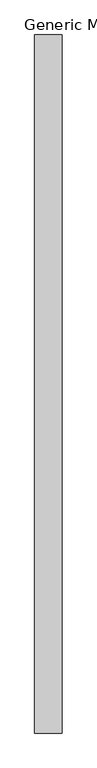
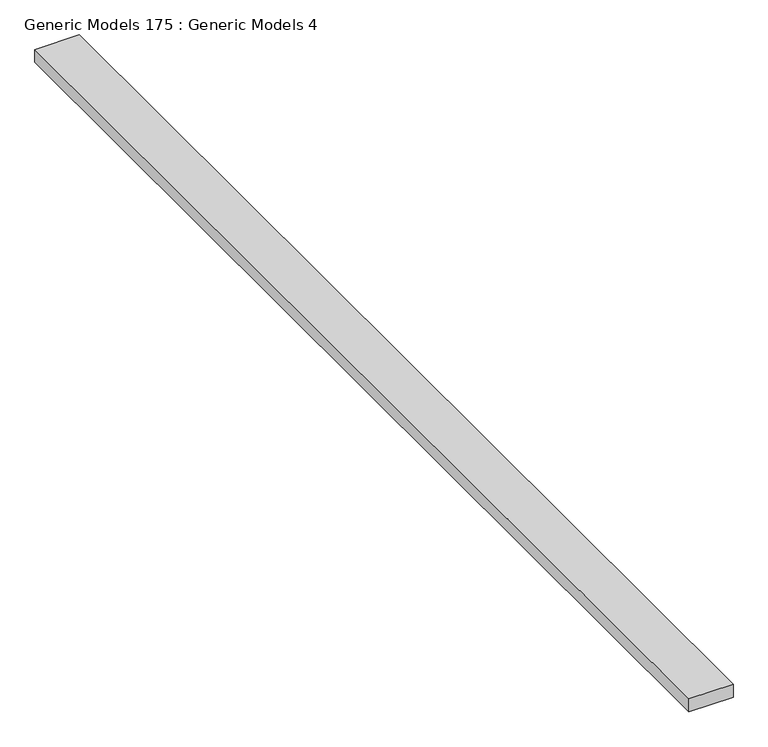
"""IFC4 building model written with IfcOpenShell, lengths in millimetres: proxy geometry, Generic Models 175 : Generic Models 4."""

from ifc_helpers import new_model, si_unit, frame, origin, place, context, project, spatial, polyline, outline, extrude, source, transform, mapped, element, save


def generic_models_175_generic_models_4_836cd898(model_context):
    return source(origin(), model_context, "Body", "SweptSolid", [
        extrude(outline(polyline([(-5937.4236296, -5493.3230338), (-6426.3736296, -5493.3230338), (-6426.3736296, 7054.2769662), (-5937.4236296, 7054.2769662), (-5937.4236296, -5493.3230338)])), frame((0.0, 0.0, 122802.396), z_axis=(0.0, 0.0, 1.0), x_axis=(1.0, 0.0, 0.0)), (0.0, 0.0, 1.0), 150.8125),
    ])


if __name__ == "__main__":
    model = new_model("IFC4")
    model_context = context("Model", 3, world=origin())
    ifc_project = project(units=[si_unit("LENGTHUNIT", "METRE", prefix="MILLI")], contexts=[model_context])
    site = spatial("IfcSite", under=ifc_project)
    building = spatial("IfcBuilding", under=site)
    placement = place(None, origin())
    generic_models_175_generic_models_4_shape = generic_models_175_generic_models_4_836cd898(model_context)
    element("IfcBuildingElementProxy", 1, Name="Generic Models 175 : Generic Models 4", ObjectType="Generic Models 175 : Generic Models 4", at=placement, inside=building, context=model_context, shape_type="MappedRepresentation", body=[
        mapped(generic_models_175_generic_models_4_shape, transform((0.0, 0.0, 0.0), x_axis=(1.0, 0.0, 0.0), y_axis=(0.0, 1.0, 0.0), z_axis=(0.0, 0.0, 1.0))),
    ])
    save(model, "model.ifc")

# Revit data of these elements
# Element 1 (IfcBuildingElementProxy, "Generic Models 175 : Generic Models 4")
#   Materials on its faces: "_COMPACTED GRADE"
# Materials
#   "_COMPACTED GRADE": class "Generic", colour RGB 120 100 58, transparency 0, Cost = 0
